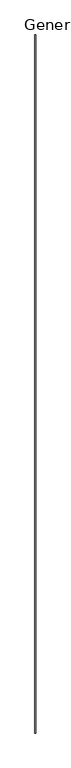
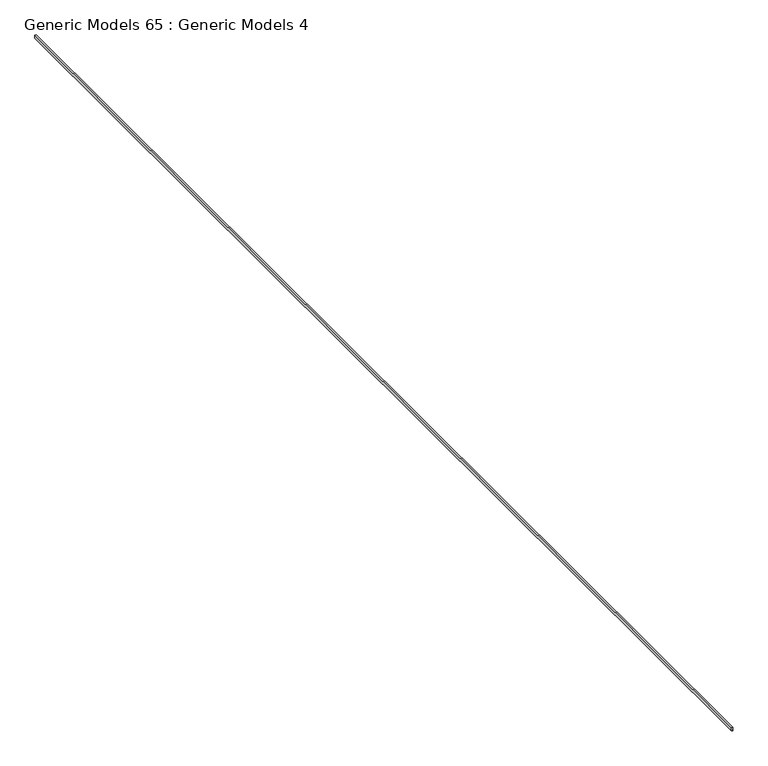
"""IFC4 building model written with IfcOpenShell, lengths in millimetres: proxy geometry, Generic Models 65 : Generic Models 4."""

from ifc_helpers import new_model, si_unit, frame, origin, place, context, project, spatial, polyline, outline, extrude, source, transform, mapped, element, save


def generic_models_65_generic_models_4_25c7cd41(model_context):
    return source(origin(), model_context, "Body", "SweptSolid", [
        extrude(outline(polyline([(126357.126, -9251.3936042), (126305.691, -9251.3936042), (126305.691, -9234.3436296), (126307.9008, -9234.3436296), (126307.9008, -9235.2024705), (126328.2153787, -9235.2024705), (126328.2153787, -9233.9324705), (126309.1708, -9233.9324705), (126309.1708, -9233.0736296), (126353.6462, -9233.0736296), (126353.6462, -9234.3436296), (126357.126, -9234.3436296), (126357.126, -9251.3936042)])), frame((0.0, -6864.9230338, 0.0), z_axis=(0.0, 1.0, 0.0), x_axis=(0.0, 0.0, 1.0)), (0.0, 0.0, 1.0), 18643.6),
    ])


if __name__ == "__main__":
    model = new_model("IFC4")
    model_context = context("Model", 3, world=origin())
    ifc_project = project(units=[si_unit("LENGTHUNIT", "METRE", prefix="MILLI")], contexts=[model_context])
    site = spatial("IfcSite", under=ifc_project)
    building = spatial("IfcBuilding", under=site)
    placement = place(None, origin())
    generic_models_65_generic_models_4_shape = generic_models_65_generic_models_4_25c7cd41(model_context)
    element("IfcBuildingElementProxy", 1, Name="Generic Models 65 : Generic Models 4", ObjectType="Generic Models 65 : Generic Models 4", at=placement, inside=building, context=model_context, shape_type="MappedRepresentation", body=[
        mapped(generic_models_65_generic_models_4_shape, transform((0.0, 0.0, 0.0), x_axis=(1.0, 0.0, 0.0), y_axis=(0.0, 1.0, 0.0), z_axis=(0.0, 0.0, 1.0))),
    ])
    save(model, "model.ifc")

# Revit data of these elements
# Element 1 (IfcBuildingElementProxy, "Generic Models 65 : Generic Models 4")
#   Materials on its faces: "_7/8\" SMOOTH TROWEL EXTERIOR STUCCO (COLOR PER OWNER)"
# Materials
#   "_7/8\" SMOOTH TROWEL EXTERIOR STUCCO (COLOR PER OWNER)": class "Generic", colour RGB 233 233 233, transparency 0, Cost = 0
